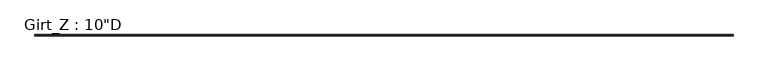
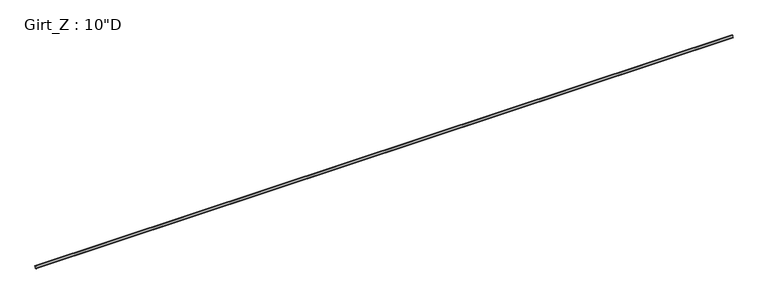
"""IFC4 building model written with IfcOpenShell, lengths in millimetres: beam geometry."""

from ifc_helpers import new_model, si_unit, point, frame, frame_2d, origin, place, context, project, spatial, polyline, circle_curve, trimmed, segment, composite_curve, outline, extrude, source, transform, mapped, element, save


def beam_f582a1bf(model_context):
    return source(origin(), model_context, "Body", "SweptSolid", [
        extrude(outline(composite_curve([segment(polyline([(63.5, 127.0), (75.745104, 112.4068534), (73.6169367, 110.621109), (62.204539, 124.221875), (3.3005807, 124.221875)]), True, "CONTINUOUS"), segment(trimmed(circle_curve(frame_2d((3.3741066, 122.2381931)), 1.9850441), [point((3.3005807, 124.221875))], [point((1.3890625, 122.2381931))], True, "CARTESIAN"), True, "CONTINUOUS"), segment(polyline([(1.3890625, 122.2381931), (1.3890625, -122.2375)]), True, "CONTINUOUS"), segment(trimmed(circle_curve(frame_2d((-3.3734375, -122.2375)), 4.7625), [point((1.3890625, -122.2375))], [point((-3.3734375, -127.0))], False, "CARTESIAN"), True, "CONTINUOUS"), segment(polyline([(-3.3734375, -127.0), (-63.5, -127.0), (-75.745104, -112.4068534), (-73.6169367, -110.621109), (-62.204539, -124.221875), (-3.2694106, -124.221875)]), True, "CONTINUOUS"), segment(trimmed(circle_curve(frame_2d((-3.3748024, -122.2389339)), 1.9857399), [point((-3.2694106, -124.221875))], [point((-1.3890625, -122.2389339))], True, "CARTESIAN"), True, "CONTINUOUS"), segment(polyline([(-1.3890625, -122.2389339), (-1.3890625, 122.2375)]), True, "CONTINUOUS"), segment(trimmed(circle_curve(frame_2d((3.3734375, 122.2375)), 4.7625), [point((-1.3890625, 122.2375))], [point((3.3734375, 127.0))], False, "CARTESIAN"), True, "CONTINUOUS"), segment(polyline([(3.3734375, 127.0), (63.5, 127.0)]), True, "CONTINUOUS")], self_intersect=False)), frame((-40443.15, 0.0, 0.0), z_axis=(1.0, 0.0, 0.0), x_axis=(0.0, 1.0, 0.0)), (0.0, 0.0, 1.0), 80886.3),
    ])


if __name__ == "__main__":
    model = new_model("IFC4")
    model_context = context("Model", 3, world=origin())
    ifc_project = project(units=[si_unit("LENGTHUNIT", "METRE", prefix="MILLI")], contexts=[model_context])
    site = spatial("IfcSite", under=ifc_project)
    building = spatial("IfcBuilding", under=site)
    placement = place(None, origin())
    beam_shape = beam_f582a1bf(model_context)
    element("IfcBeam", 1, ObjectType="Girt_Z : 10\"D", at=placement, inside=building, context=model_context, shape_type="MappedRepresentation", body=[
        mapped(beam_shape, transform((0.0, 0.0, 0.0), x_axis=(1.0, 0.0, 0.0), y_axis=(0.0, 1.0, 0.0), z_axis=(0.0, 0.0, 1.0))),
    ])
    save(model, "model.ifc")

# Revit data of these elements
# Type "Girt_Z : 10\"D"
#   Web_Thickness = 0' - 0 7/64"
#   Length [instance default] = 10' - 0"
#   Leg_1 = 0' - 2 1/2"
#   Height = 0' - 10"
#   Structural Material [instance default] = none
